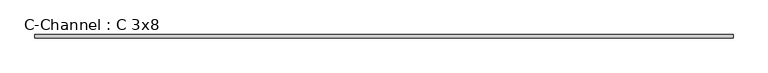
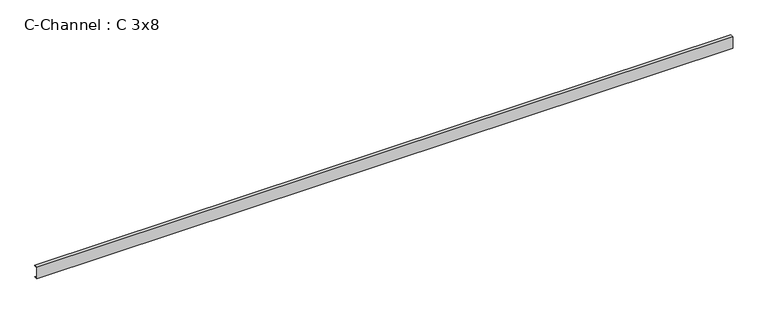
"""IFC4 building model written with IfcOpenShell, lengths in millimetres: beam geometry, C-Channel : C 3x8."""

from ifc_helpers import new_model, si_unit, point, frame, frame_2d, origin, place, context, project, spatial, polyline, circle_curve, trimmed, segment, composite_curve, outline, extrude, source, transform, mapped, element, save


def c_channel_c_3x8_b0b678fc(model_context):
    return source(origin(), model_context, "Body", "SweptSolid", [
        extrude(outline(composite_curve([segment(polyline([(-13.5128, 101.6), (44.9072, 101.6)]), True, "CONTINUOUS"), segment(trimmed(circle_curve(frame_2d((35.6108, 101.6)), 9.2964), [point((44.9072, 101.6))], [point((35.6108, 92.3036))], False, "CARTESIAN"), True, "CONTINUOUS"), segment(polyline([(35.6108, 92.3036), (-2.8702, 86.2088084), (-2.8702, -86.2088084), (35.6108, -92.3036)]), True, "CONTINUOUS"), segment(trimmed(circle_curve(frame_2d((35.6108, -101.6)), 9.2964), [point((35.6108, -92.3036))], [point((44.9072, -101.6))], False, "CARTESIAN"), True, "CONTINUOUS"), segment(polyline([(44.9072, -101.6), (-13.5128, -101.6), (-13.5128, 101.6)]), True, "CONTINUOUS")], self_intersect=False)), frame((-5835.65, 0.0, 0.0), z_axis=(1.0, 0.0, 0.0), x_axis=(0.0, 1.0, 0.0)), (0.0, 0.0, 1.0), 11671.2999994),
    ])


if __name__ == "__main__":
    model = new_model("IFC4")
    model_context = context("Model", 3, world=origin())
    ifc_project = project(units=[si_unit("LENGTHUNIT", "METRE", prefix="MILLI")], contexts=[model_context])
    site = spatial("IfcSite", under=ifc_project)
    building = spatial("IfcBuilding", under=site)
    placement = place(None, origin())
    c_channel_c_3x8_shape = c_channel_c_3x8_b0b678fc(model_context)
    element("IfcBeam", 1, ObjectType="C-Channel : C 3x8", at=placement, inside=building, context=model_context, shape_type="MappedRepresentation", body=[
        mapped(c_channel_c_3x8_shape, transform((0.0, 0.0, 0.0), x_axis=(1.0, 0.0, 0.0), y_axis=(0.0, 1.0, 0.0), z_axis=(0.0, 0.0, 1.0))),
    ])
    save(model, "model.ifc")

# Revit data of these elements
# Type "C-Channel : C 3x8"
#   Assembly Code = "B10"
#   W = 14.7
#   Length [instance default] = 5' - 0"
#   bf = 0' - 2.3"
#   d = 0' - 8"
#   tf = 0' - 0.366"
#   tw = 0' - 0.419"
#   x = 0' - 0.532"
#   A = 0.0300694 SF
#   Structural Material [instance default] = Steel ASTM A36
# Element 1 (IfcBeam, "C-Channel : C 3x8")
#   Structural Material = Steel ASTM A992
#   Materials on its faces: "Steel ASTM A992"
# Materials
#   "Steel ASTM A36": class "Metal", colour RGB 199 199 199, transparency 0, Description = "Structural steel, ASTM A36 Grade B, mill finish", Cost = 0
#   "Steel ASTM A992": class "Metal", colour RGB 189 187 185, transparency 0, Description = "Structural steel 50ksi", Cost = 0
